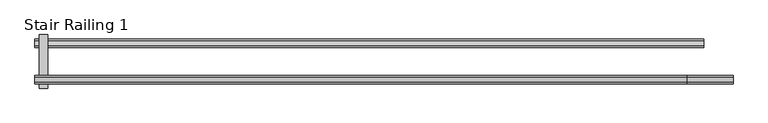
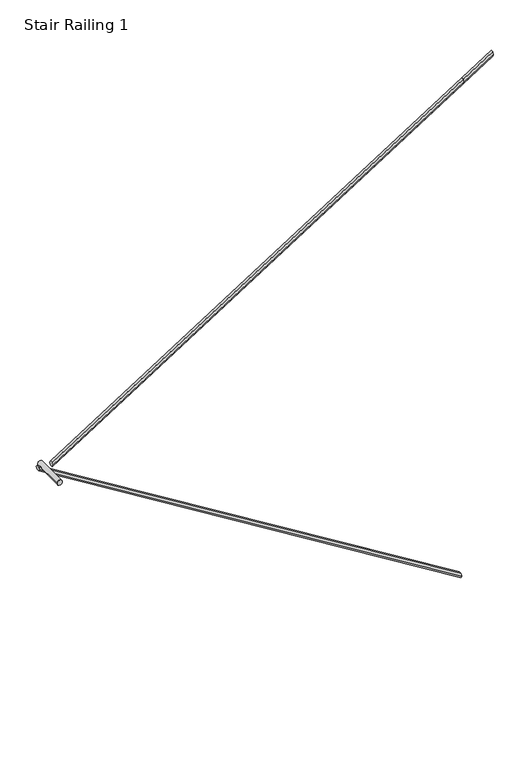
"""IFC4 building model written with IfcOpenShell, lengths in millimetres: railing geometry, Stair Railing 1."""

import ifcopenshell
import ifcopenshell.guid

model = None  # the IFC model being written
_history = None  # IfcOwnerHistory: only IFC2X3 demands one
_inside = {}  # id of a spatial element -> (the spatial element, [elements in it])
_under = {}  # id of a project, library or spatial element -> (it, [spatial elements below it])
_declared = {}  # id of a project -> (the project, [libraries it declares])
_typed = {}  # id of a type object -> (the type object, [elements of that type])
_made_of = {}  # id of a material, layer set ... -> (it, [elements and type objects made of it])


def new_model(schema):
    """Start an empty IFC model of exactly this schema.

    Asked for "IFC4X3", IfcOpenShell would pick the latest addendum, in which some entities
    have other attributes; the version numbers below select the first issue.
    IFC2X3 requires an IfcOwnerHistory on every rooted entity: one is made here for all.
    """
    global model, _history
    if schema == "IFC4X3":
        model = ifcopenshell.file(schema_version=(4, 3, 0, 0))
    else:
        model = ifcopenshell.file(schema=schema)
    _inside.clear()
    _under.clear()
    _declared.clear()
    _typed.clear()
    _made_of.clear()
    _history = None
    if model.schema == "IFC2X3":
        org = make("IfcOrganization", Name="unknown")
        user = make(
            "IfcPersonAndOrganization",
            ThePerson=make("IfcPerson", FamilyName="unknown"),
            TheOrganization=org,
        )
        app = make(
            "IfcApplication",
            ApplicationDeveloper=org,
            Version="unknown",
            ApplicationFullName="unknown",
            ApplicationIdentifier="unknown",
        )
        _history = make(
            "IfcOwnerHistory",
            OwningUser=user,
            OwningApplication=app,
            ChangeAction="ADDED",
            CreationDate=0,
        )
    return model


def make(cls, **values):
    """One entity of the class cls with the attributes given. An attribute that is None is left unset."""
    return model.create_entity(
        cls, **{name: value for name, value in values.items() if value is not None}
    )


def rooted(cls, **values):
    """An entity with a GlobalId (a new one), such as an element, a storey or a relation."""
    return make(cls, GlobalId=ifcopenshell.guid.new(), OwnerHistory=_history, **values)


def si_unit(unit_type, name, prefix=None):
    """IfcSIUnit, for example si_unit("LENGTHUNIT", "METRE", prefix="MILLI")."""
    return make("IfcSIUnit", UnitType=unit_type, Prefix=prefix, Name=name)


def assignment(units):
    """IfcUnitAssignment: the units of a project."""
    return None if units is None else make("IfcUnitAssignment", Units=units)


def point(xyz):
    """IfcCartesianPoint."""
    return None if xyz is None else make("IfcCartesianPoint", Coordinates=xyz)


def direction(xyz):
    """IfcDirection."""
    return None if xyz is None else make("IfcDirection", DirectionRatios=xyz)


def frame(location, z_axis=None, x_axis=None):
    """IfcAxis2Placement3D, a coordinate frame: its origin and axes. An axis left out is left unset."""
    return make(
        "IfcAxis2Placement3D",
        Location=point(location),
        Axis=direction(z_axis),
        RefDirection=direction(x_axis),
    )


def origin():
    """The frame at (0, 0, 0) with its axes left unset."""
    return frame((0.0, 0.0, 0.0))


def place(relative_to, where):
    """IfcLocalPlacement: puts the frame where relative to a parent placement (None: the world)."""
    return make(
        "IfcLocalPlacement", PlacementRelTo=relative_to, RelativePlacement=where
    )


def context(
    kind, dimensions, precision=None, world=None, true_north=None, identifier=None
):
    """IfcGeometricRepresentationContext, for example the 3D "Model" context."""
    return make(
        "IfcGeometricRepresentationContext",
        ContextIdentifier=identifier,
        ContextType=kind,
        CoordinateSpaceDimension=dimensions,
        Precision=precision,
        WorldCoordinateSystem=world,
        TrueNorth=true_north,
    )


def project(units=None, contexts=None):
    """IfcProject with its units and contexts."""
    return rooted(
        "IfcProject",
        Name="project",
        RepresentationContexts=contexts,
        UnitsInContext=assignment(units),
    )


def spatial(cls, under=None, at=None, **own):
    """A site, building, storey or space (cls), placed at a placement, below another one or the project."""
    s = rooted(cls, ObjectPlacement=at, **own)
    if under is not None:
        _under.setdefault(under.id(), (under, []))[1].append(s)
    return s


def circle_curve(where, radius):
    """IfcCircle in the frame where."""
    return make("IfcCircle", Position=where, Radius=radius)


def faces_of(points, faces, orient=None, outer=None):
    """IfcFace entities. A face is a list of loops; a loop is a list of indices into points, from 0.

    orient and outer hold one flag for each loop. By default every Orientation is true, the
    first loop of a face is its IfcFaceOuterBound and the others are IfcFaceBound.
    """
    made = []
    for i, loops in enumerate(faces):
        bounds = []
        for j, loop in enumerate(loops):
            is_outer = j == 0 if outer is None else outer[i][j]
            bounds.append(
                make(
                    "IfcFaceOuterBound" if is_outer else "IfcFaceBound",
                    Bound=make("IfcPolyLoop", Polygon=[points[k] for k in loop]),
                    Orientation=True if orient is None else orient[i][j],
                )
            )
        made.append(make("IfcFace", Bounds=bounds))
    return made


def faceted_brep(points, faces, orient=None, outer=None, voids=None):
    """IfcFacetedBrep: a solid bounded by flat faces; with voids (closed shells), ...WithVoids."""
    shared = [point(p) for p in points]
    hull = make("IfcClosedShell", CfsFaces=faces_of(shared, faces, orient, outer))
    if voids is None:
        return make("IfcFacetedBrep", Outer=hull)
    return make(
        "IfcFacetedBrepWithVoids",
        Outer=hull,
        Voids=[
            make(cls, CfsFaces=faces_of(shared, fs, o, b)) for cls, fs, o, b in voids
        ],
    )


def shape(context_of_items, identifier, shape_type, items):
    """IfcShapeRepresentation: the items that make up one representation, for example the "Body"."""
    return make(
        "IfcShapeRepresentation",
        ContextOfItems=context_of_items,
        RepresentationIdentifier=identifier,
        RepresentationType=shape_type,
        Items=items,
    )


def source(mapping_origin, context_of_items, identifier, shape_type, items):
    """IfcRepresentationMap: a shape defined once, which mapped items show again and again."""
    return make(
        "IfcRepresentationMap",
        MappingOrigin=mapping_origin,
        MappedRepresentation=shape(context_of_items, identifier, shape_type, items),
    )


def transform(
    local_origin,
    x_axis=None,
    y_axis=None,
    z_axis=None,
    scale=None,
    scale2=None,
    scale3=None,
    uniform=True,
):
    """IfcCartesianTransformationOperator3D, or its non-uniform kind. x_axis, y_axis, z_axis: its Axis1, 2, 3."""
    if uniform:
        return make(
            "IfcCartesianTransformationOperator3D",
            Axis1=direction(x_axis),
            Axis2=direction(y_axis),
            LocalOrigin=point(local_origin),
            Scale=scale,
            Axis3=direction(z_axis),
        )
    return make(
        "IfcCartesianTransformationOperator3DnonUniform",
        Axis1=direction(x_axis),
        Axis2=direction(y_axis),
        LocalOrigin=point(local_origin),
        Scale=scale,
        Axis3=direction(z_axis),
        Scale2=scale2,
        Scale3=scale3,
    )


def mapped(mapping_source, mapping_target):
    """IfcMappedItem: shows the shape of a source again, moved by a transform."""
    return make(
        "IfcMappedItem", MappingSource=mapping_source, MappingTarget=mapping_target
    )


def made_of(thing, what):
    """Note that an element or type object is made of a material, layer set ...; save() writes the relation."""
    if what is not None:
        _made_of.setdefault(what.id(), (what, []))[1].append(thing)
    return thing


def element(
    cls,
    number,
    at=None,
    inside=None,
    cuts=None,
    type_object=None,
    material=None,
    context=None,
    identifier="Body",
    shape_type=None,
    held_by="IfcProductDefinitionShape",
    body=None,
    shapes=None,
    **own,
):
    """One element of the class cls, such as IfcWall. Its Tag is "e" and its number.

    at: its placement. inside: the storey or other place that contains it. cuts: it is an
    opening in that element (IfcRelVoidsElement). A single representation is given by context,
    identifier, shape_type and body (its items); several are given by shapes. held_by: the class
    of the entity that holds the representations. save() writes the other relations.
    """
    e = rooted(cls, Tag="e%d" % number, ObjectPlacement=at, **own)
    if body is not None:
        shapes = [shape(context, identifier, shape_type, body)]
    if shapes is not None:
        e.Representation = make(held_by, Representations=shapes)
    if inside is not None:
        _inside.setdefault(inside.id(), (inside, []))[1].append(e)
    if cuts is not None:
        rooted(
            "IfcRelVoidsElement", RelatingBuildingElement=cuts, RelatedOpeningElement=e
        )
    if type_object is not None:
        _typed.setdefault(type_object.id(), (type_object, []))[1].append(e)
    return made_of(e, material)


def aggregate(whole, parts):
    """IfcRelAggregates: a whole, such as a stair, and the parts it consists of."""
    return rooted("IfcRelAggregates", RelatingObject=whole, RelatedObjects=parts)


def save(model, path):
    """Write the relations noted so far, then the file.

    IfcRelAggregates (storeys below a building ...), IfcRelContainedInSpatialStructure (elements
    in a storey), IfcRelDefinesByType, IfcRelAssociatesMaterial and IfcRelDeclares: one each for
    every whole, place, type object, material and project.
    """
    for whole, parts in _under.values():
        aggregate(whole, parts)
    for where, things in _inside.values():
        rooted(
            "IfcRelContainedInSpatialStructure",
            RelatedElements=things,
            RelatingStructure=where,
        )
    for kind, things in _typed.values():
        rooted("IfcRelDefinesByType", RelatedObjects=things, RelatingType=kind)
    for what, things in _made_of.values():
        rooted("IfcRelAssociatesMaterial", RelatedObjects=things, RelatingMaterial=what)
    for by, libraries in _declared.values():
        rooted("IfcRelDeclares", RelatingContext=by, RelatedDefinitions=libraries)
    model.write(path)


def plane_surface(at):
    """IfcPlane: the flat surface through the origin of the frame at, square to its z axis."""
    return make("IfcPlane", Position=at)


def cylinder_surface(at, radius):
    """IfcCylindricalSurface: all points at the distance radius from the z axis of the frame at."""
    return make("IfcCylindricalSurface", Position=at, Radius=radius)


def advanced_brep(points, edges, surfaces, faces):
    """IfcAdvancedBrep: a solid bounded by faces that lie on surfaces and meet in shared edges.

    An edge is (start, end): straight between two places in points (the first is 0);
    or (start, end, curve); or (start, end, curve, False) where it runs against its curve.
    A face is (place in surfaces, loops), or (place, loops, False) where it looks against
    its surface's normal. A loop lists edges by number (the first is 1), with a minus sign
    where the edge is run from its end to its start. The first loop is the outer one.
    """
    corners = [point(p) for p in points]
    vertices = [make("IfcVertexPoint", VertexGeometry=c) for c in corners]
    made = []
    for start, end, *more in edges:
        made.append(
            make(
                "IfcEdgeCurve",
                EdgeStart=vertices[start],
                EdgeEnd=vertices[end],
                EdgeGeometry=more[0] if more else make("IfcPolyline", Points=[corners[start], corners[end]]),
                SameSense=more[1] if len(more) > 1 else True,
            )
        )
    hull = []
    for where, loops, *sense in faces:
        bounds = []
        for j, loop in enumerate(loops):
            ring = [make("IfcOrientedEdge", EdgeElement=made[abs(k) - 1], Orientation=k > 0) for k in loop]
            bounds.append(
                make(
                    "IfcFaceOuterBound" if j == 0 else "IfcFaceBound",
                    Bound=make("IfcEdgeLoop", EdgeList=ring),
                    Orientation=True,
                )
            )
        hull.append(make("IfcAdvancedFace", Bounds=bounds, FaceSurface=surfaces[where], SameSense=sense[0] if sense else True))
    return make("IfcAdvancedBrep", Outer=make("IfcClosedShell", CfsFaces=hull))


def stair_railing_1_19f522ab(model_context):
    return source(origin(), model_context, "Body", "SolidModel", [
        faceted_brep([(46517.5398084, 46191.4865351, 3746.9096774), (46517.5398084, 46204.1865351, 3768.9067227), (46517.5398084, 46229.5865351, 3768.9067227), (46517.5398084, 46242.2865351, 3746.9096774), (46517.5398084, 46229.5865351, 3724.9126322), (46517.5398084, 46204.1865351, 3724.9126322), (50533.2139908, 46191.4865351, 1269.1806452), (50533.2139908, 46204.1865351, 1247.1835999), (50533.2139908, 46229.5865351, 1247.1835999), (50533.2139908, 46242.2865351, 1269.1806452), (50533.2139908, 46229.5865351, 1291.1776904), (50533.2139908, 46204.1865351, 1291.1776904)], [[[0, 1, 2, 3, 4, 5]], [[6, 7, 8, 9, 10, 11]], [[1, 0, 6, 11]], [[2, 1, 11, 10]], [[3, 2, 10, 9]], [[4, 3, 9, 8]], [[5, 4, 8, 7]], [[0, 5, 7, 6]]]),
        advanced_brep(
        [(46593.7398084, 45946.4030566, 3746.9096774), (46542.9398084, 45946.4030566, 3746.9096774), (46593.7398084, 46267.6865351, 3746.9096774), (46542.9398084, 46267.6865351, 3746.9096774)],
        [
            (0, 1, circle_curve(frame((46568.3398084, 45946.4030566, 3746.9096774), z_axis=(0.0, -1.0, 0.0), x_axis=(1.0, 0.0, 0.0)), 25.4)),
            (1, 0, circle_curve(frame((46568.3398084, 45946.4030566, 3746.9096774), z_axis=(0.0, -1.0, 0.0), x_axis=(1.0, 0.0, 0.0)), 25.4)),
            (2, 3, circle_curve(frame((46568.3398084, 46267.6865351, 3746.9096774), z_axis=(0.0, 1.0, 0.0), x_axis=(1.0, 0.0, 0.0)), 25.4)),
            (3, 2, circle_curve(frame((46568.3398084, 46267.6865351, 3746.9096774), z_axis=(0.0, 1.0, 0.0), x_axis=(1.0, 0.0, 0.0)), 25.4)),
            (0, 2),
            (3, 1),
        ],
        [
            plane_surface(frame((46593.7398084, 45946.4030566, 3721.5096774), z_axis=(0.0, -1.0, 0.0), x_axis=(0.0, 0.0, -1.0))),
            plane_surface(frame((46593.7398084, 46267.6865351, 3721.5096774), z_axis=(0.0, 1.0, 0.0), x_axis=(0.0, 0.0, 1.0))),
            cylinder_surface(frame((46568.3398084, 46267.6865351, 3746.9096774), z_axis=(0.0, -1.0, 0.0), x_axis=(1.0, 0.0, 0.0)), 25.4),
        ],
        [
            (0, [[1, 2]]),
            (1, [[3, 4]]),
            (2, [[-1, 5, -4, 6]]),
            (2, [[-2, -6, -3, -5]]),
        ],
    ),
        faceted_brep([(50429.1398084, 46022.6030566, 6401.6193548), (50429.1398084, 46009.9030566, 6423.6164001), (50429.1398084, 45984.5030566, 6423.6164001), (50429.1398084, 45971.8030566, 6401.6193548), (50429.1398084, 45984.5030566, 6379.6223096), (50429.1398084, 46009.9030566, 6379.6223096), (46517.5398084, 46022.6030566, 3923.8903226), (46517.5398084, 46009.9030566, 3901.8932773), (46517.5398084, 45984.5030566, 3901.8932773), (46517.5398084, 45971.8030566, 3923.8903226), (46517.5398084, 45984.5030566, 3945.8873678), (46517.5398084, 46009.9030566, 3945.8873678)], [[[0, 1, 2, 3, 4, 5]], [[6, 7, 8, 9, 10, 11]], [[1, 0, 6, 11]], [[2, 1, 11, 10]], [[3, 2, 10, 9]], [[4, 3, 9, 8]], [[5, 4, 8, 7]], [[0, 5, 7, 6]]]),
        faceted_brep([(50708.5398084, 46022.6030566, 6578.6), (50708.5398084, 46009.9030566, 6600.5970453), (50708.5398084, 45984.5030566, 6600.5970453), (50708.5398084, 45971.8030566, 6578.6), (50708.5398084, 45984.5030566, 6556.6029547), (50708.5398084, 46009.9030566, 6556.6029547), (50429.1398084, 46022.6030566, 6401.6193548), (50429.1398084, 46009.9030566, 6379.6223096), (50429.1398084, 45984.5030566, 6379.6223096), (50429.1398084, 45971.8030566, 6401.6193548), (50429.1398084, 45984.5030566, 6423.6164001), (50429.1398084, 46009.9030566, 6423.6164001)], [[[0, 1, 2, 3, 4, 5]], [[6, 7, 8, 9, 10, 11]], [[1, 0, 6, 11]], [[2, 1, 11, 10]], [[3, 2, 10, 9]], [[4, 3, 9, 8]], [[5, 4, 8, 7]], [[0, 5, 7, 6]]]),
    ])


if __name__ == "__main__":
    model = new_model("IFC4")
    model_context = context("Model", 3, world=origin())
    ifc_project = project(units=[si_unit("LENGTHUNIT", "METRE", prefix="MILLI")], contexts=[model_context])
    site = spatial("IfcSite", under=ifc_project)
    building = spatial("IfcBuilding", under=site)
    placement = place(None, origin())
    stair_railing_1_shape = stair_railing_1_19f522ab(model_context)
    element("IfcRailing", 1, ObjectType="Stair Railing 1", at=placement, inside=building, context=model_context, shape_type="MappedRepresentation", body=[
        mapped(stair_railing_1_shape, transform((0.0, 0.0, 0.0), x_axis=(1.0, 0.0, 0.0), y_axis=(0.0, 1.0, 0.0), z_axis=(0.0, 0.0, 1.0))),
    ])
    save(model, "model.ifc")
